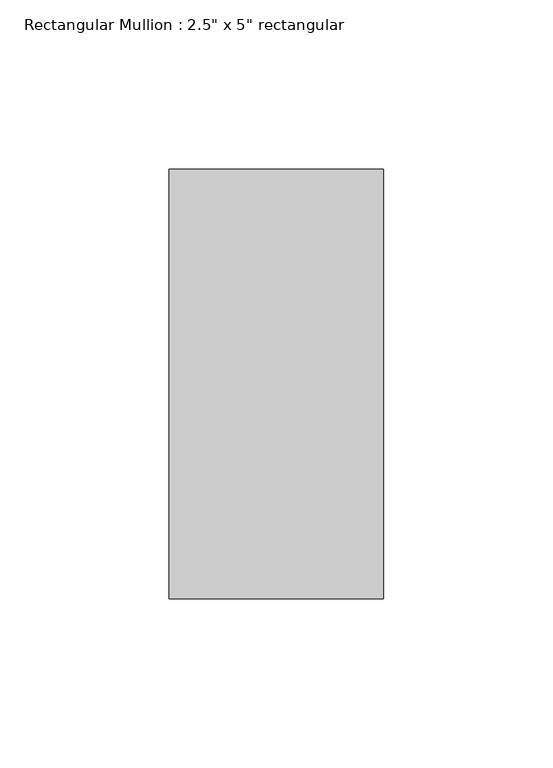
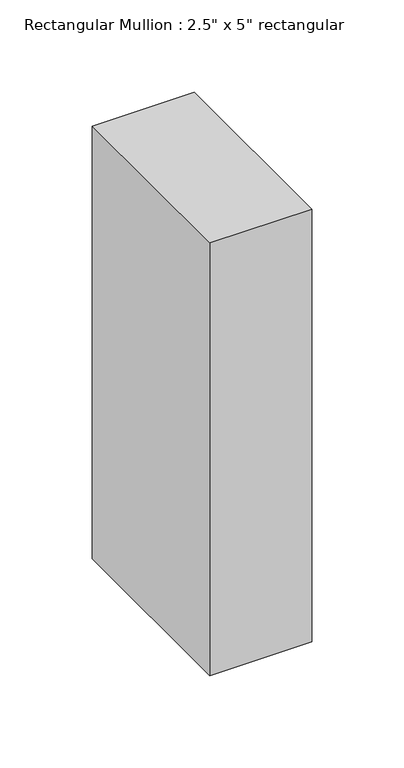
"""IFC4 building model written with IfcOpenShell, lengths in millimetres: member geometry."""

from ifc_helpers import new_model, si_unit, frame, origin, place, context, project, spatial, polyline, outline, extrude, source, transform, mapped, element, save


def member_dff87739(model_context):
    return source(origin(), model_context, "Body", "SweptSolid", [
        extrude(outline(polyline([(31.75, 63.5), (31.75, -63.5), (-31.75, -63.5), (-31.75, 63.5), (31.75, 63.5)])), frame((0.0, 0.0, -285.75), z_axis=(0.0, 0.0, 1.0), x_axis=(1.0, 0.0, 0.0)), (0.0, 0.0, 1.0), 285.75),
    ])


if __name__ == "__main__":
    model = new_model("IFC4")
    model_context = context("Model", 3, world=origin())
    ifc_project = project(units=[si_unit("LENGTHUNIT", "METRE", prefix="MILLI")], contexts=[model_context])
    site = spatial("IfcSite", under=ifc_project)
    building = spatial("IfcBuilding", under=site)
    placement = place(None, origin())
    member_shape = member_dff87739(model_context)
    element("IfcMember", 1, ObjectType="Rectangular Mullion : 2.5\" x 5\" rectangular", at=placement, inside=building, context=model_context, shape_type="MappedRepresentation", body=[
        mapped(member_shape, transform((0.0, 0.0, 0.0), x_axis=(1.0, 0.0, 0.0), y_axis=(0.0, 1.0, 0.0), z_axis=(0.0, 0.0, 1.0))),
    ])
    save(model, "model.ifc")

# Revit data of these elements
# Type "Rectangular Mullion : 2.5\" x 5\" rectangular"
#   built-in parameter 1007304 = 0.416667 (stored number, unit not read)
#   built-in parameter 1007301 = 0.104167 (stored number, unit not read)
#   built-in parameter 1007300 = 0.104167 (stored number, unit not read)
# Element 1 (IfcMember, "Rectangular Mullion : 2.5\" x 5\" rectangular")
#   Materials on its faces: "Metal - Aluminum"
# Materials
#   "Metal - Aluminum": class "Metal", colour RGB 140 140 140, transparency 0
